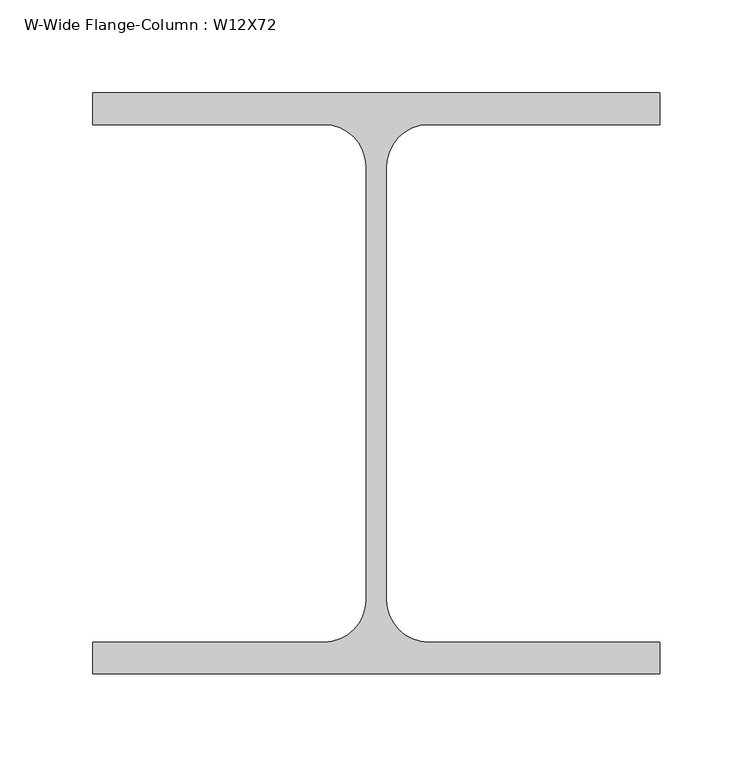
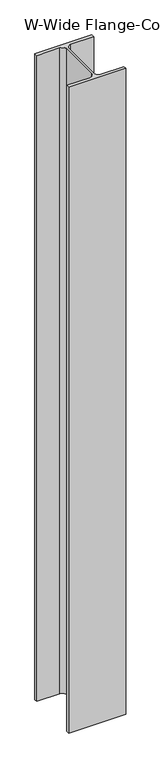
"""IFC4 building model written with IfcOpenShell, lengths in millimetres: column geometry, W-Wide Flange-Column : W12X72."""

from ifc_helpers import new_model, si_unit, point, frame, frame_2d, origin, place, context, project, spatial, polyline, circle_curve, trimmed, segment, composite_curve, outline, extrude, source, transform, mapped, element, save


def w_wide_flange_column_w12x72_cab3a303(model_context):
    return source(origin(), model_context, "Body", "SweptSolid", [
        extrude(outline(composite_curve([segment(polyline([(152.4, 156.21), (152.4, 139.192), (28.1305, 139.192)]), True, "CONTINUOUS"), segment(trimmed(circle_curve(frame_2d((28.1305, 116.5225)), 22.6695), [point((28.1305, 139.192))], [point((5.461, 116.5225))], True, "CARTESIAN"), True, "CONTINUOUS"), segment(polyline([(5.461, 116.5225), (5.461, -116.5225)]), True, "CONTINUOUS"), segment(trimmed(circle_curve(frame_2d((28.1305, -116.5225)), 22.6695), [point((5.461, -116.5225))], [point((28.1305, -139.192))], True, "CARTESIAN"), True, "CONTINUOUS"), segment(polyline([(28.1305, -139.192), (152.4, -139.192), (152.4, -156.21), (-152.4, -156.21), (-152.4, -139.192), (-28.1305, -139.192)]), True, "CONTINUOUS"), segment(trimmed(circle_curve(frame_2d((-28.1305, -116.5225)), 22.6695), [point((-28.1305, -139.192))], [point((-5.461, -116.5225))], True, "CARTESIAN"), True, "CONTINUOUS"), segment(polyline([(-5.461, -116.5225), (-5.461, 116.5225)]), True, "CONTINUOUS"), segment(trimmed(circle_curve(frame_2d((-28.1305, 116.5225)), 22.6695), [point((-5.461, 116.5225))], [point((-28.1305, 139.192))], True, "CARTESIAN"), True, "CONTINUOUS"), segment(polyline([(-28.1305, 139.192), (-152.4, 139.192), (-152.4, 156.21), (152.4, 156.21)]), True, "CONTINUOUS")], self_intersect=False)), frame((0.0, 0.0, 8756.65), z_axis=(0.0, 0.0, 1.0), x_axis=(1.0, 0.0, 0.0)), (0.0, 0.0, 1.0), 3651.25),
    ])


if __name__ == "__main__":
    model = new_model("IFC4")
    model_context = context("Model", 3, world=origin())
    ifc_project = project(units=[si_unit("LENGTHUNIT", "METRE", prefix="MILLI")], contexts=[model_context])
    site = spatial("IfcSite", under=ifc_project)
    building = spatial("IfcBuilding", under=site)
    placement = place(None, origin())
    w_wide_flange_column_w12x72_shape = w_wide_flange_column_w12x72_cab3a303(model_context)
    element("IfcColumn", 1, ObjectType="W-Wide Flange-Column : W12X72", at=placement, inside=building, context=model_context, shape_type="MappedRepresentation", body=[
        mapped(w_wide_flange_column_w12x72_shape, transform((0.0, 0.0, 0.0), x_axis=(1.0, 0.0, 0.0), y_axis=(0.0, 1.0, 0.0), z_axis=(0.0, 0.0, 1.0))),
    ])
    save(model, "model.ifc")

# Revit data of these elements
# Type "W-Wide Flange-Column : W12X72"
#   Assembly Code = "B10"
#   W = 72
#   bf = 1' - 0"
#   d = 1' - 0.3"
#   k = 0' - 1 9/16"
#   kr = 0' - 0.8925"
#   tf = 0' - 0.67"
#   tw = 0' - 0.43"
#   A = 0.146528 SF
#   Structural Material [instance default] = Steel ASTM A992
# Element 1 (IfcColumn, "W-Wide Flange-Column : W12X72")
#   Materials on its faces: "Steel ASTM A992"
# Materials
#   "Steel ASTM A992": class "Metal", colour RGB 199 199 199, transparency 0, Description = "Structural steel 50ksi", Cost = 0
